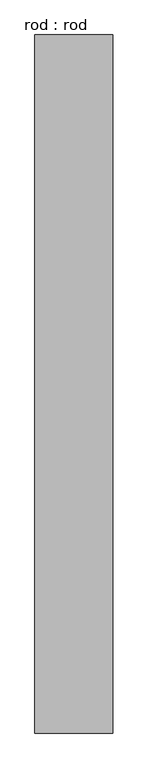
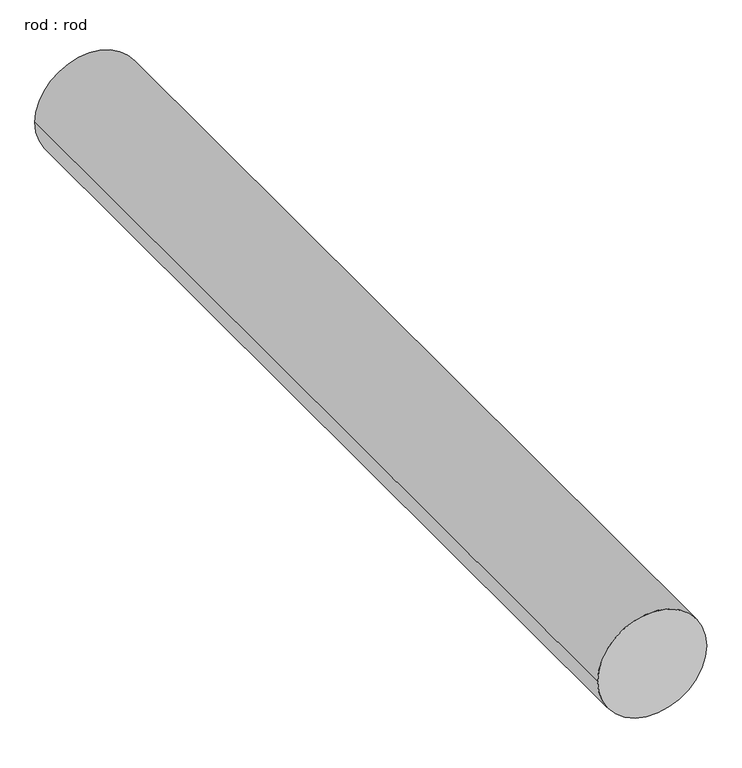
"""IFC4 building model written with IfcOpenShell, lengths in millimetres: proxy geometry, rod : rod."""

from ifc_helpers import new_model, si_unit, point, frame, frame_2d, origin, place, context, project, spatial, circle_curve, trimmed, segment, composite_curve, outline, extrude, source, transform, mapped, element, save


def rod_rod_066012d8(model_context):
    return source(origin(), model_context, "Body", "SweptSolid", [
        extrude(outline(composite_curve([segment(trimmed(circle_curve(frame_2d((0.0108462, 0.0)), 200.0), [point((0.0108462, 200.0))], [point((0.0108462, -200.0))], False, "CARTESIAN"), True, "CONTINUOUS"), segment(trimmed(circle_curve(frame_2d((0.0108462, 0.0)), 200.0), [point((0.0108462, -200.0))], [point((0.0108462, 200.0))], False, "CARTESIAN"), True, "CONTINUOUS")], self_intersect=False)), frame((0.0, 2302.7286153, 0.0), z_axis=(0.0, 1.0, 0.0), x_axis=(0.0, 0.0, 1.0)), (0.0, 0.0, 1.0), 3580.0),
    ])


if __name__ == "__main__":
    model = new_model("IFC4")
    model_context = context("Model", 3, world=origin())
    ifc_project = project(units=[si_unit("LENGTHUNIT", "METRE", prefix="MILLI")], contexts=[model_context])
    site = spatial("IfcSite", under=ifc_project)
    building = spatial("IfcBuilding", under=site)
    placement = place(None, origin())
    rod_rod_shape = rod_rod_066012d8(model_context)
    element("IfcBuildingElementProxy", 1, Name="rod : rod", ObjectType="rod : rod", at=placement, inside=building, context=model_context, shape_type="MappedRepresentation", body=[
        mapped(rod_rod_shape, transform((0.0, 0.0, 0.0), x_axis=(1.0, 0.0, 0.0), y_axis=(0.0, 1.0, 0.0), z_axis=(0.0, 0.0, 1.0))),
    ])
    save(model, "model.ifc")

# Revit data of these elements
# Type "rod : rod"
#   Default Elevation = 0
